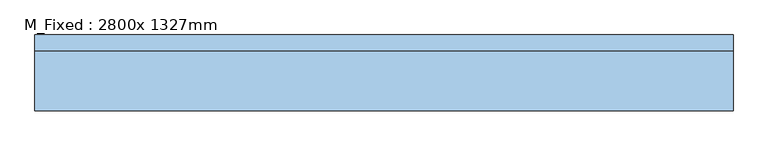
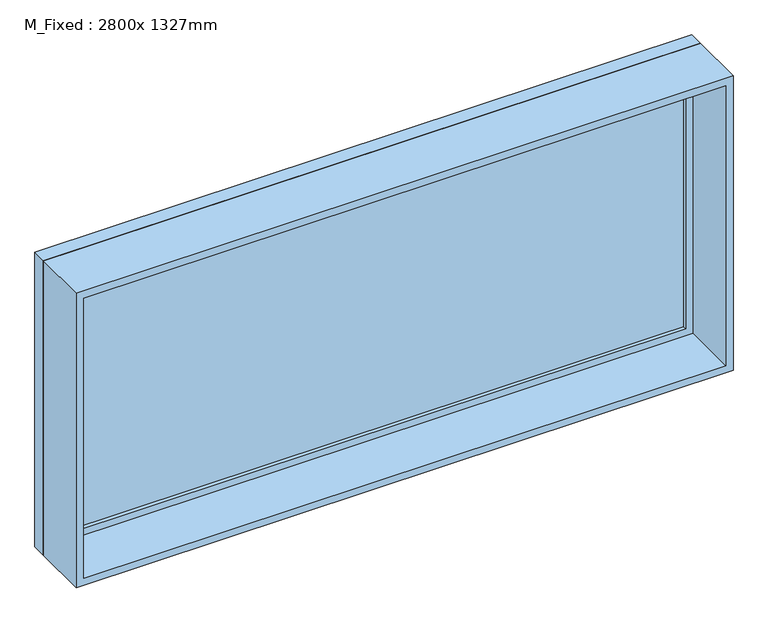
"""IFC4 building model written with IfcOpenShell, lengths in millimetres: window geometry, M_Fixed : 2800x 1327mm."""

from ifc_helpers import new_model, si_unit, frame, origin, place, context, project, spatial, polyline, outline, extrude, source, transform, mapped, element, save


def m_fixed_2800x_1327mm_376a1ccb(model_context):
    return source(origin(), model_context, "Body", "SweptSolid", [
        extrude(outline(polyline([(-1337.0, 130.4), (1337.0, 130.4), (1337.0, 118.4), (-1337.0, 118.4), (-1337.0, 130.4)])), frame((0.0, 0.0, 978.0), z_axis=(0.0, 0.0, 1.0), x_axis=(1.0, 0.0, 0.0)), (0.0, 0.0, 1.0), 1201.2),
        extrude(outline(polyline([(2223.2, -1381.0), (934.0, -1381.0), (934.0, 1381.0), (2223.2, 1381.0), (2223.2, -1381.0)]), holes=[polyline([(2179.2, -1337.0), (2179.2, 1337.0), (978.0, 1337.0), (978.0, -1337.0), (2179.2, -1337.0)])]), frame((0.0, 102.4, 0.0), z_axis=(0.0, 1.0, 0.0), x_axis=(0.0, 0.0, 1.0)), (0.0, 0.0, 1.0), 44.0),
        extrude(outline(polyline([(2242.2, -1400.0), (915.0, -1400.0), (915.0, 1400.0), (2242.2, 1400.0), (2242.2, -1400.0)]), holes=[polyline([(2223.2, -1381.0), (2223.2, 1381.0), (934.0, 1381.0), (934.0, -1381.0), (2223.2, -1381.0)])]), frame((0.0, 102.4, 0.0), z_axis=(0.0, 1.0, 0.0), x_axis=(0.0, 0.0, 1.0)), (0.0, 0.0, 1.0), 63.0),
        extrude(outline(polyline([(2242.2, -1400.0), (915.0, -1400.0), (915.0, 1400.0), (2242.2, 1400.0), (2242.2, -1400.0)]), holes=[polyline([(2210.2, -1368.0), (2210.2, 1368.0), (947.0, 1368.0), (947.0, -1368.0), (2210.2, -1368.0)])]), frame((0.0, -139.4, 0.0), z_axis=(0.0, 1.0, 0.0), x_axis=(0.0, 0.0, 1.0)), (0.0, 0.0, 1.0), 241.8),
    ])


if __name__ == "__main__":
    model = new_model("IFC4")
    model_context = context("Model", 3, world=origin())
    ifc_project = project(units=[si_unit("LENGTHUNIT", "METRE", prefix="MILLI")], contexts=[model_context])
    site = spatial("IfcSite", under=ifc_project)
    building = spatial("IfcBuilding", under=site)
    placement = place(None, origin())
    m_fixed_2800x_1327mm_shape = m_fixed_2800x_1327mm_376a1ccb(model_context)
    element("IfcWindow", 1, ObjectType="M_Fixed : 2800x 1327mm", at=placement, inside=building, context=model_context, shape_type="MappedRepresentation", body=[
        mapped(m_fixed_2800x_1327mm_shape, transform((0.0, 0.0, 0.0), x_axis=(1.0, 0.0, 0.0), y_axis=(0.0, 1.0, 0.0), z_axis=(0.0, 0.0, 1.0))),
    ])
    save(model, "model.ifc")

# Revit data of these elements
# Type "M_Fixed : 2800x 1327mm"
#   Type Mark = "46"
#   Height = 1327.2 mm
#   Default Sill Height = 915 mm
#   Width = 2800 mm
#   Window Inset = 19 mm
#   Frame Exterior Material = Sash
#   Frame Interior Material = Sash
#   Glass Pane Material = Glass
#   Sash = Sash
#   Wall Closure = (empty or 0)
# Element 1 (IfcWindow, "M_Fixed : 2800x 1327mm")
#   Materials on its faces: "Sash", "Glass"
# Materials
#   "Sash": class "Wood", colour RGB 136 99 55, transparency 0
#   "Glass": class "Glass", colour RGB 0 128 192, transparency 0.9, Description = "Soda Lime Glass", Cost = 0
